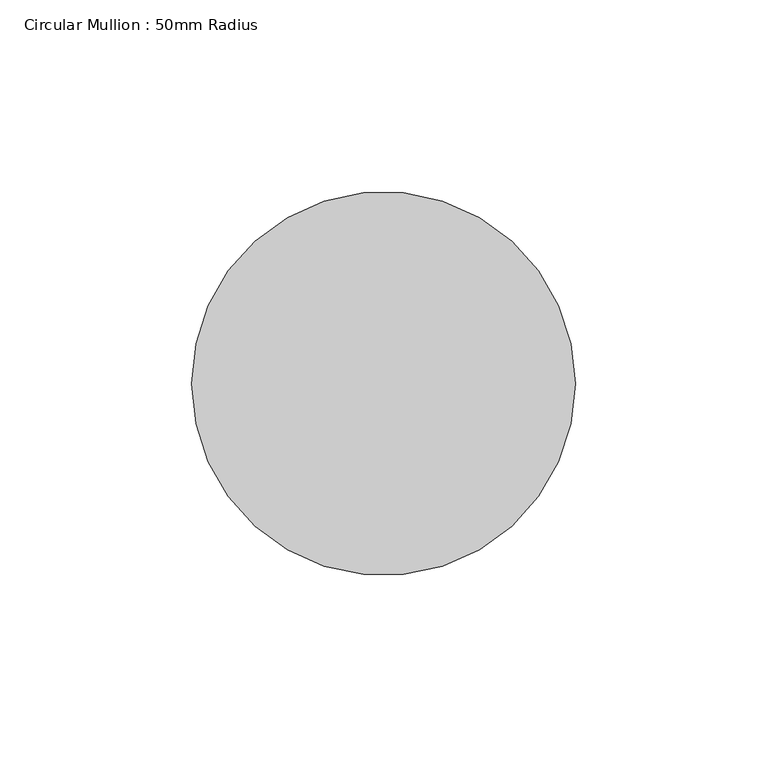
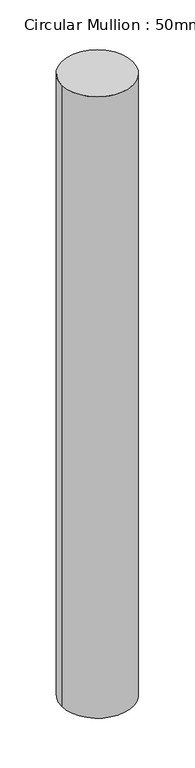
"""IFC4 building model written with IfcOpenShell, lengths in millimetres: member geometry, Circular Mullion : 50mm Radius."""

from ifc_helpers import new_model, si_unit, point, frame, origin, origin_2d, place, context, project, spatial, circle_curve, trimmed, segment, composite_curve, outline, extrude, source, transform, mapped, element, save


def circular_mullion_50mm_radius_b67505a2(model_context):
    return source(origin(), model_context, "Body", "SweptSolid", [
        extrude(outline(composite_curve([segment(trimmed(circle_curve(origin_2d(), 50.0), [point((50.0, 0.0))], [point((-50.0, 0.0))], False, "CARTESIAN"), True, "CONTINUOUS"), segment(trimmed(circle_curve(origin_2d(), 50.0), [point((-50.0, 0.0))], [point((50.0, 0.0))], False, "CARTESIAN"), True, "CONTINUOUS")], self_intersect=False)), frame((0.0, 0.0, -922.2839785), z_axis=(0.0, 0.0, 1.0), x_axis=(1.0, 0.0, 0.0)), (0.0, 0.0, 1.0), 922.2839785),
    ])


if __name__ == "__main__":
    model = new_model("IFC4")
    model_context = context("Model", 3, world=origin())
    ifc_project = project(units=[si_unit("LENGTHUNIT", "METRE", prefix="MILLI")], contexts=[model_context])
    site = spatial("IfcSite", under=ifc_project)
    building = spatial("IfcBuilding", under=site)
    placement = place(None, origin())
    circular_mullion_50mm_radius_shape = circular_mullion_50mm_radius_b67505a2(model_context)
    element("IfcMember", 1, ObjectType="Circular Mullion : 50mm Radius", at=placement, inside=building, context=model_context, shape_type="MappedRepresentation", body=[
        mapped(circular_mullion_50mm_radius_shape, transform((0.0, 0.0, 0.0), x_axis=(1.0, 0.0, 0.0), y_axis=(0.0, 1.0, 0.0), z_axis=(0.0, 0.0, 1.0))),
    ])
    save(model, "model.ifc")

# Revit data of these elements
# Type "Circular Mullion : 50mm Radius"
#   built-in parameter 1007350 = 0.164042 (stored number, unit not read)
# Element 1 (IfcMember, "Circular Mullion : 50mm Radius")
#   Materials on its faces: "Aluminium"
# Materials
#   "Aluminium": class "Metal", colour RGB 247 247 247, transparency 0, Description = "Aluminium 6061", Cost = 0
